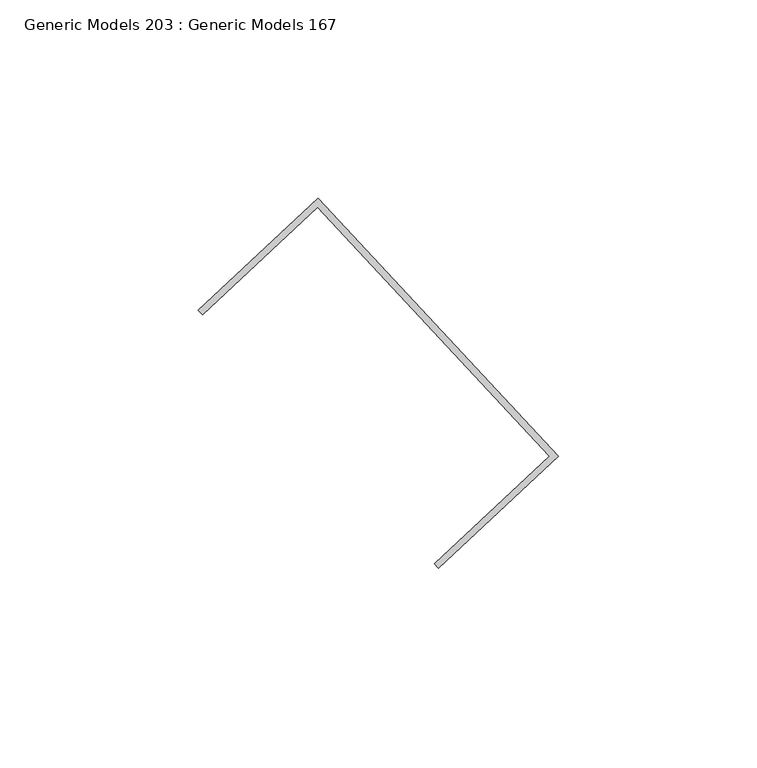
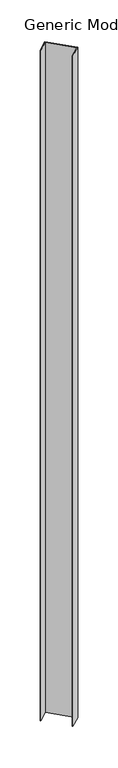
"""IFC4 building model written with IfcOpenShell, lengths in millimetres: proxy geometry, Generic Models 203 : Generic Models 167."""

from ifc_helpers import new_model, si_unit, origin, origin_with_axes, place, context, project, spatial, polyline, outline, extrude, source, transform, mapped, element, save


def generic_models_203_generic_models_167_8a07fe50(model_context):
    return source(origin(), model_context, "Body", "SweptSolid", [
        extrude(outline(polyline([(58486.5460698, 3594.5988566), (58457.5204698, 3567.5320466), (58456.4377974, 3568.6930706), (58486.6244214, 3596.842553), (58547.2540756, 3531.8252089), (58517.0674516, 3503.6757266), (58515.9847792, 3504.8367506), (58545.0103792, 3531.9035605), (58486.5460698, 3594.5988566)])), origin_with_axes(), (0.0, 0.0, 1.0), 2133.6),
    ])


if __name__ == "__main__":
    model = new_model("IFC4")
    model_context = context("Model", 3, world=origin())
    ifc_project = project(units=[si_unit("LENGTHUNIT", "METRE", prefix="MILLI")], contexts=[model_context])
    site = spatial("IfcSite", under=ifc_project)
    building = spatial("IfcBuilding", under=site)
    placement = place(None, origin())
    generic_models_203_generic_models_167_shape = generic_models_203_generic_models_167_8a07fe50(model_context)
    element("IfcBuildingElementProxy", 1, Name="Generic Models 203 : Generic Models 167", ObjectType="Generic Models 203 : Generic Models 167", at=placement, inside=building, context=model_context, shape_type="MappedRepresentation", body=[
        mapped(generic_models_203_generic_models_167_shape, transform((0.0, 0.0, 0.0), x_axis=(1.0, 0.0, 0.0), y_axis=(0.0, 1.0, 0.0), z_axis=(0.0, 0.0, 1.0))),
    ])
    save(model, "model.ifc")

# Revit data of these elements
# Element 1 (IfcBuildingElementProxy, "Generic Models 203 : Generic Models 167")
#   Materials on its faces: "EXISTING STOREFRONT"
# Materials
#   "EXISTING STOREFRONT": class "Metal", colour RGB 244 244 244, transparency 0, Description = "Aluminum 6061", Cost = 0
